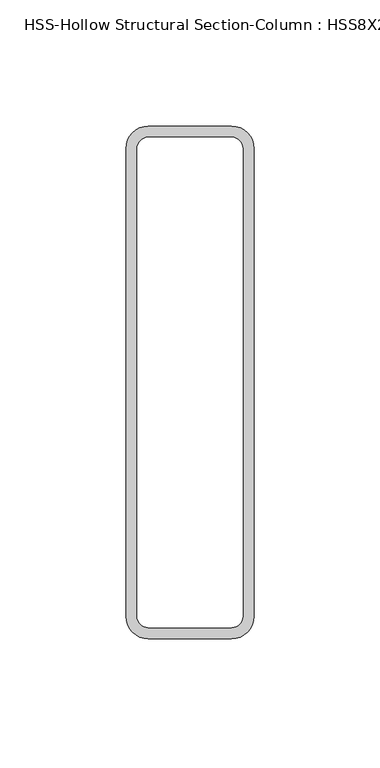
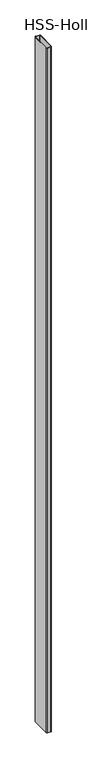
"""IFC4 building model written with IfcOpenShell, lengths in millimetres: column geometry, HSS-Hollow Structural Section-Column : HSS8X2X3/16."""

from ifc_helpers import new_model, si_unit, point, frame, frame_2d, origin, place, context, project, spatial, polyline, circle_curve, trimmed, segment, composite_curve, outline, extrude, source, transform, mapped, element, save


def hss_hollow_structural_section_column_hss8x2x3_16_3803074a(model_context):
    return source(origin(), model_context, "Body", "SweptSolid", [
        extrude(outline(composite_curve([segment(trimmed(circle_curve(frame_2d((16.5608, 92.7608)), 8.8392), [point((16.5608, 101.6))], [point((25.4, 92.7608))], False, "CARTESIAN"), True, "CONTINUOUS"), segment(polyline([(25.4, 92.7608), (25.4, -92.7608)]), True, "CONTINUOUS"), segment(trimmed(circle_curve(frame_2d((16.5608, -92.7608)), 8.8392), [point((25.4, -92.7608))], [point((16.5608, -101.6))], False, "CARTESIAN"), True, "CONTINUOUS"), segment(polyline([(16.5608, -101.6), (-16.5608, -101.6)]), True, "CONTINUOUS"), segment(trimmed(circle_curve(frame_2d((-16.5608, -92.7608)), 8.8392), [point((-16.5608, -101.6))], [point((-25.4, -92.7608))], False, "CARTESIAN"), True, "CONTINUOUS"), segment(polyline([(-25.4, -92.7608), (-25.4, 92.7608)]), True, "CONTINUOUS"), segment(trimmed(circle_curve(frame_2d((-16.5608, 92.7608)), 8.8392), [point((-25.4, 92.7608))], [point((-16.5608, 101.6))], False, "CARTESIAN"), True, "CONTINUOUS"), segment(polyline([(-16.5608, 101.6), (16.5608, 101.6)]), True, "CONTINUOUS")], self_intersect=False), holes=[composite_curve([segment(polyline([(16.5608, 97.1804), (-16.5608, 97.1804)]), True, "CONTINUOUS"), segment(trimmed(circle_curve(frame_2d((-16.5608, 92.7608)), 4.4196), [point((-16.5608, 97.1804))], [point((-20.9804, 92.7608))], True, "CARTESIAN"), True, "CONTINUOUS"), segment(polyline([(-20.9804, 92.7608), (-20.9804, -92.7608)]), True, "CONTINUOUS"), segment(trimmed(circle_curve(frame_2d((-16.5608, -92.7608)), 4.4196), [point((-20.9804, -92.7608))], [point((-16.5608, -97.1804))], True, "CARTESIAN"), True, "CONTINUOUS"), segment(polyline([(-16.5608, -97.1804), (16.5608, -97.1804)]), True, "CONTINUOUS"), segment(trimmed(circle_curve(frame_2d((16.5608, -92.7608)), 4.4196), [point((16.5608, -97.1804))], [point((20.9804, -92.7608))], True, "CARTESIAN"), True, "CONTINUOUS"), segment(polyline([(20.9804, -92.7608), (20.9804, 92.7608)]), True, "CONTINUOUS"), segment(trimmed(circle_curve(frame_2d((16.5608, 92.7608)), 4.4196), [point((20.9804, 92.7608))], [point((16.5608, 97.1804))], True, "CARTESIAN"), True, "CONTINUOUS")], self_intersect=False)]), frame((0.0, 0.0, -1200.0), z_axis=(0.0, 0.0, 1.0), x_axis=(1.0, 0.0, 0.0)), (0.0, 0.0, 1.0), 7205.0),
    ])


if __name__ == "__main__":
    model = new_model("IFC4")
    model_context = context("Model", 3, world=origin())
    ifc_project = project(units=[si_unit("LENGTHUNIT", "METRE", prefix="MILLI")], contexts=[model_context])
    site = spatial("IfcSite", under=ifc_project)
    building = spatial("IfcBuilding", under=site)
    placement = place(None, origin())
    hss_hollow_structural_section_column_hss8x2x3_16_shape = hss_hollow_structural_section_column_hss8x2x3_16_3803074a(model_context)
    element("IfcColumn", 1, ObjectType="HSS-Hollow Structural Section-Column : HSS8X2X3/16", at=placement, inside=building, context=model_context, shape_type="MappedRepresentation", body=[
        mapped(hss_hollow_structural_section_column_hss8x2x3_16_shape, transform((0.0, 0.0, 0.0), x_axis=(1.0, 0.0, 0.0), y_axis=(0.0, 1.0, 0.0), z_axis=(0.0, 0.0, 1.0))),
    ])
    save(model, "model.ifc")

# Revit data of these elements
# Type "HSS-Hollow Structural Section-Column : HSS8X2X3/16"
#   Assembly Code = "B10"
#   Shape = "Rect."
#   Cost = 1
#   W = 12
#   Ht = 203.2 mm
#   b = 50.8 mm
#   kr = 8.839 mm
#   t = 4.42 mm
#   A = 0.00211612 m²
#   Structural Material [instance default] = Steel ASTM A500, Grade B, Rectangular and Square
# Element 1 (IfcColumn, "HSS-Hollow Structural Section-Column : HSS8X2X3/16")
#   Structural Material = Metal - Steel 43-275
#   Materials on its faces: "Metal - Steel 43-275"
# Materials
#   "Steel ASTM A500, Grade B, Rectangular and Square": class "Metal", colour RGB 199 199 199, transparency 0, Description = "Carbon steel", Cost = 0
#   "Metal - Steel 43-275": class "Metal", colour RGB 247 247 247, transparency 0, Cost = 0
